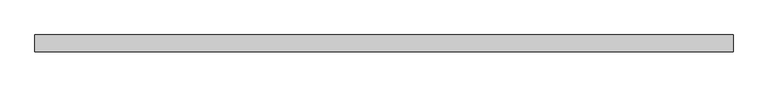
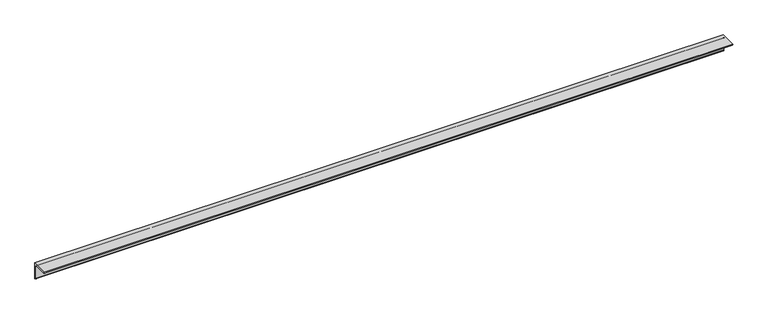
"""IFC4 building model written with IfcOpenShell, lengths in millimetres: member geometry, 0912_Steel Framing_L-KSD3502 : H_SB_AR_S03_L-130x130x12_HBR3."""

import ifcopenshell
import ifcopenshell.guid

model = None  # the IFC model being written
_history = None  # IfcOwnerHistory: only IFC2X3 demands one
_inside = {}  # id of a spatial element -> (the spatial element, [elements in it])
_under = {}  # id of a project, library or spatial element -> (it, [spatial elements below it])
_declared = {}  # id of a project -> (the project, [libraries it declares])
_typed = {}  # id of a type object -> (the type object, [elements of that type])
_made_of = {}  # id of a material, layer set ... -> (it, [elements and type objects made of it])


def new_model(schema):
    """Start an empty IFC model of exactly this schema.

    Asked for "IFC4X3", IfcOpenShell would pick the latest addendum, in which some entities
    have other attributes; the version numbers below select the first issue.
    IFC2X3 requires an IfcOwnerHistory on every rooted entity: one is made here for all.
    """
    global model, _history
    if schema == "IFC4X3":
        model = ifcopenshell.file(schema_version=(4, 3, 0, 0))
    else:
        model = ifcopenshell.file(schema=schema)
    _inside.clear()
    _under.clear()
    _declared.clear()
    _typed.clear()
    _made_of.clear()
    _history = None
    if model.schema == "IFC2X3":
        org = make("IfcOrganization", Name="unknown")
        user = make(
            "IfcPersonAndOrganization",
            ThePerson=make("IfcPerson", FamilyName="unknown"),
            TheOrganization=org,
        )
        app = make(
            "IfcApplication",
            ApplicationDeveloper=org,
            Version="unknown",
            ApplicationFullName="unknown",
            ApplicationIdentifier="unknown",
        )
        _history = make(
            "IfcOwnerHistory",
            OwningUser=user,
            OwningApplication=app,
            ChangeAction="ADDED",
            CreationDate=0,
        )
    return model


def make(cls, **values):
    """One entity of the class cls with the attributes given. An attribute that is None is left unset."""
    return model.create_entity(
        cls, **{name: value for name, value in values.items() if value is not None}
    )


def rooted(cls, **values):
    """An entity with a GlobalId (a new one), such as an element, a storey or a relation."""
    return make(cls, GlobalId=ifcopenshell.guid.new(), OwnerHistory=_history, **values)


def si_unit(unit_type, name, prefix=None):
    """IfcSIUnit, for example si_unit("LENGTHUNIT", "METRE", prefix="MILLI")."""
    return make("IfcSIUnit", UnitType=unit_type, Prefix=prefix, Name=name)


def assignment(units):
    """IfcUnitAssignment: the units of a project."""
    return None if units is None else make("IfcUnitAssignment", Units=units)


def point(xyz):
    """IfcCartesianPoint."""
    return None if xyz is None else make("IfcCartesianPoint", Coordinates=xyz)


def direction(xyz):
    """IfcDirection."""
    return None if xyz is None else make("IfcDirection", DirectionRatios=xyz)


def frame(location, z_axis=None, x_axis=None):
    """IfcAxis2Placement3D, a coordinate frame: its origin and axes. An axis left out is left unset."""
    return make(
        "IfcAxis2Placement3D",
        Location=point(location),
        Axis=direction(z_axis),
        RefDirection=direction(x_axis),
    )


def frame_2d(location, x_axis=None):
    """IfcAxis2Placement2D, a coordinate frame in the plane: its origin and x axis."""
    return make(
        "IfcAxis2Placement2D", Location=point(location), RefDirection=direction(x_axis)
    )


def origin():
    """The frame at (0, 0, 0) with its axes left unset."""
    return frame((0.0, 0.0, 0.0))


def place(relative_to, where):
    """IfcLocalPlacement: puts the frame where relative to a parent placement (None: the world)."""
    return make(
        "IfcLocalPlacement", PlacementRelTo=relative_to, RelativePlacement=where
    )


def context(
    kind, dimensions, precision=None, world=None, true_north=None, identifier=None
):
    """IfcGeometricRepresentationContext, for example the 3D "Model" context."""
    return make(
        "IfcGeometricRepresentationContext",
        ContextIdentifier=identifier,
        ContextType=kind,
        CoordinateSpaceDimension=dimensions,
        Precision=precision,
        WorldCoordinateSystem=world,
        TrueNorth=true_north,
    )


def project(units=None, contexts=None):
    """IfcProject with its units and contexts."""
    return rooted(
        "IfcProject",
        Name="project",
        RepresentationContexts=contexts,
        UnitsInContext=assignment(units),
    )


def spatial(cls, under=None, at=None, **own):
    """A site, building, storey or space (cls), placed at a placement, below another one or the project."""
    s = rooted(cls, ObjectPlacement=at, **own)
    if under is not None:
        _under.setdefault(under.id(), (under, []))[1].append(s)
    return s


def polyline(points):
    """IfcPolyline through the points."""
    return make("IfcPolyline", Points=[point(p) for p in points])


def circle_curve(where, radius):
    """IfcCircle in the frame where."""
    return make("IfcCircle", Position=where, Radius=radius)


def trimmed(basis, trim1, trim2, sense, master):
    """IfcTrimmedCurve: the piece of a basis curve between two trims."""
    return make(
        "IfcTrimmedCurve",
        BasisCurve=basis,
        Trim1=trim1,
        Trim2=trim2,
        SenseAgreement=sense,
        MasterRepresentation=master,
    )


def segment(curve, same_sense, transition):
    """IfcCompositeCurveSegment."""
    return make(
        "IfcCompositeCurveSegment",
        Transition=transition,
        SameSense=same_sense,
        ParentCurve=curve,
    )


def composite_curve(segments, self_intersect=None):
    """IfcCompositeCurve: segments joined end to end."""
    return make("IfcCompositeCurve", Segments=segments, SelfIntersect=self_intersect)


def outline(outer, holes=None, kind="AREA"):
    """IfcArbitraryClosedProfileDef: a profile drawn as a closed curve; with holes, ...WithVoids."""
    if holes is None:
        return make("IfcArbitraryClosedProfileDef", ProfileType=kind, OuterCurve=outer)
    return make(
        "IfcArbitraryProfileDefWithVoids",
        ProfileType=kind,
        OuterCurve=outer,
        InnerCurves=holes,
    )


def extrude(swept, where, along, depth):
    """IfcExtrudedAreaSolid: the profile swept, set in the frame where, extruded along a direction by depth."""
    return make(
        "IfcExtrudedAreaSolid",
        SweptArea=swept,
        Position=where,
        ExtrudedDirection=direction(along),
        Depth=depth,
    )


def shape(context_of_items, identifier, shape_type, items):
    """IfcShapeRepresentation: the items that make up one representation, for example the "Body"."""
    return make(
        "IfcShapeRepresentation",
        ContextOfItems=context_of_items,
        RepresentationIdentifier=identifier,
        RepresentationType=shape_type,
        Items=items,
    )


def source(mapping_origin, context_of_items, identifier, shape_type, items):
    """IfcRepresentationMap: a shape defined once, which mapped items show again and again."""
    return make(
        "IfcRepresentationMap",
        MappingOrigin=mapping_origin,
        MappedRepresentation=shape(context_of_items, identifier, shape_type, items),
    )


def transform(
    local_origin,
    x_axis=None,
    y_axis=None,
    z_axis=None,
    scale=None,
    scale2=None,
    scale3=None,
    uniform=True,
):
    """IfcCartesianTransformationOperator3D, or its non-uniform kind. x_axis, y_axis, z_axis: its Axis1, 2, 3."""
    if uniform:
        return make(
            "IfcCartesianTransformationOperator3D",
            Axis1=direction(x_axis),
            Axis2=direction(y_axis),
            LocalOrigin=point(local_origin),
            Scale=scale,
            Axis3=direction(z_axis),
        )
    return make(
        "IfcCartesianTransformationOperator3DnonUniform",
        Axis1=direction(x_axis),
        Axis2=direction(y_axis),
        LocalOrigin=point(local_origin),
        Scale=scale,
        Axis3=direction(z_axis),
        Scale2=scale2,
        Scale3=scale3,
    )


def mapped(mapping_source, mapping_target):
    """IfcMappedItem: shows the shape of a source again, moved by a transform."""
    return make(
        "IfcMappedItem", MappingSource=mapping_source, MappingTarget=mapping_target
    )


def made_of(thing, what):
    """Note that an element or type object is made of a material, layer set ...; save() writes the relation."""
    if what is not None:
        _made_of.setdefault(what.id(), (what, []))[1].append(thing)
    return thing


def element(
    cls,
    number,
    at=None,
    inside=None,
    cuts=None,
    type_object=None,
    material=None,
    context=None,
    identifier="Body",
    shape_type=None,
    held_by="IfcProductDefinitionShape",
    body=None,
    shapes=None,
    **own,
):
    """One element of the class cls, such as IfcWall. Its Tag is "e" and its number.

    at: its placement. inside: the storey or other place that contains it. cuts: it is an
    opening in that element (IfcRelVoidsElement). A single representation is given by context,
    identifier, shape_type and body (its items); several are given by shapes. held_by: the class
    of the entity that holds the representations. save() writes the other relations.
    """
    e = rooted(cls, Tag="e%d" % number, ObjectPlacement=at, **own)
    if body is not None:
        shapes = [shape(context, identifier, shape_type, body)]
    if shapes is not None:
        e.Representation = make(held_by, Representations=shapes)
    if inside is not None:
        _inside.setdefault(inside.id(), (inside, []))[1].append(e)
    if cuts is not None:
        rooted(
            "IfcRelVoidsElement", RelatingBuildingElement=cuts, RelatedOpeningElement=e
        )
    if type_object is not None:
        _typed.setdefault(type_object.id(), (type_object, []))[1].append(e)
    return made_of(e, material)


def aggregate(whole, parts):
    """IfcRelAggregates: a whole, such as a stair, and the parts it consists of."""
    return rooted("IfcRelAggregates", RelatingObject=whole, RelatedObjects=parts)


def save(model, path):
    """Write the relations noted so far, then the file.

    IfcRelAggregates (storeys below a building ...), IfcRelContainedInSpatialStructure (elements
    in a storey), IfcRelDefinesByType, IfcRelAssociatesMaterial and IfcRelDeclares: one each for
    every whole, place, type object, material and project.
    """
    for whole, parts in _under.values():
        aggregate(whole, parts)
    for where, things in _inside.values():
        rooted(
            "IfcRelContainedInSpatialStructure",
            RelatedElements=things,
            RelatingStructure=where,
        )
    for kind, things in _typed.values():
        rooted("IfcRelDefinesByType", RelatedObjects=things, RelatingType=kind)
    for what, things in _made_of.values():
        rooted("IfcRelAssociatesMaterial", RelatedObjects=things, RelatingMaterial=what)
    for by, libraries in _declared.values():
        rooted("IfcRelDeclares", RelatingContext=by, RelatedDefinitions=libraries)
    model.write(path)


def member_6cc94826(model_context):
    return source(origin(), model_context, "Body", "SweptSolid", [
        extrude(outline(composite_curve([segment(polyline([(36.4, 36.4), (36.4, -93.6)]), True, "CONTINUOUS"), segment(trimmed(circle_curve(frame_2d((36.4, -81.6)), 12.0), [point((36.4, -93.6))], [point((24.4, -81.6))], False, "CARTESIAN"), True, "CONTINUOUS"), segment(polyline([(24.4, -81.6), (24.4, 12.4)]), True, "CONTINUOUS"), segment(trimmed(circle_curve(frame_2d((12.4, 12.4)), 12.0), [point((24.4, 12.4))], [point((12.4, 24.4))], True, "CARTESIAN"), True, "CONTINUOUS"), segment(polyline([(12.4, 24.4), (-81.6, 24.4)]), True, "CONTINUOUS"), segment(trimmed(circle_curve(frame_2d((-81.6, 36.4)), 12.0), [point((-81.6, 24.4))], [point((-93.6, 36.4))], False, "CARTESIAN"), True, "CONTINUOUS"), segment(polyline([(-93.6, 36.4), (36.4, 36.4)]), True, "CONTINUOUS")], self_intersect=False)), frame((-2682.0951934, 0.0, 0.0), z_axis=(1.0, 0.0, 0.0), x_axis=(0.0, 1.0, 0.0)), (0.0, 0.0, 1.0), 5417.5661112),
    ])


if __name__ == "__main__":
    model = new_model("IFC4")
    model_context = context("Model", 3, world=origin())
    ifc_project = project(units=[si_unit("LENGTHUNIT", "METRE", prefix="MILLI")], contexts=[model_context])
    site = spatial("IfcSite", under=ifc_project)
    building = spatial("IfcBuilding", under=site)
    placement = place(None, origin())
    member_shape = member_6cc94826(model_context)
    element("IfcMember", 1, ObjectType="0912_Steel Framing_L-KSD3502 : H_SB_AR_S03_L-130x130x12_HBR3", at=placement, inside=building, context=model_context, shape_type="MappedRepresentation", body=[
        mapped(member_shape, transform((0.0, 0.0, 0.0), x_axis=(1.0, 0.0, 0.0), y_axis=(0.0, 1.0, 0.0), z_axis=(0.0, 0.0, 1.0))),
    ])
    save(model, "model.ifc")

# Revit data of these elements
# Type "0912_Steel Framing_L-KSD3502 : H_SB_AR_S03_L-130x130x12_HBR3"
#   k = 25 mm
#   Perimeter = 0.52 m²/m
#   Nominal Weight = 23.40 kgf/m
#   Length [instance default] = 1000 mm
#   b = 130 mm
#   d = 130 mm
#   t = 12 mm
#   x = 36.4 mm
#   y = 36.4 mm
#   A = 2976.00 m²
#   Structural Material [instance default] = Steel, 45-345
# Element 1 (IfcMember, "0912_Steel Framing_L-KSD3502 : H_SB_AR_S03_L-130x130x12_HBR3")
#   Structural Material = Steel ASTM A36
#   Materials on its faces: "Steel ASTM A36"
# Materials
#   "Steel, 45-345": class "Metal", colour RGB 189 187 185, transparency 0, Description = "Steel 345 MPa", Cost = 0
#   "Steel ASTM A36": class "Metal", colour RGB 199 199 199, transparency 0, Description = "Structural steel, ASTM A36 Grade B, mill finish", Cost = 0
